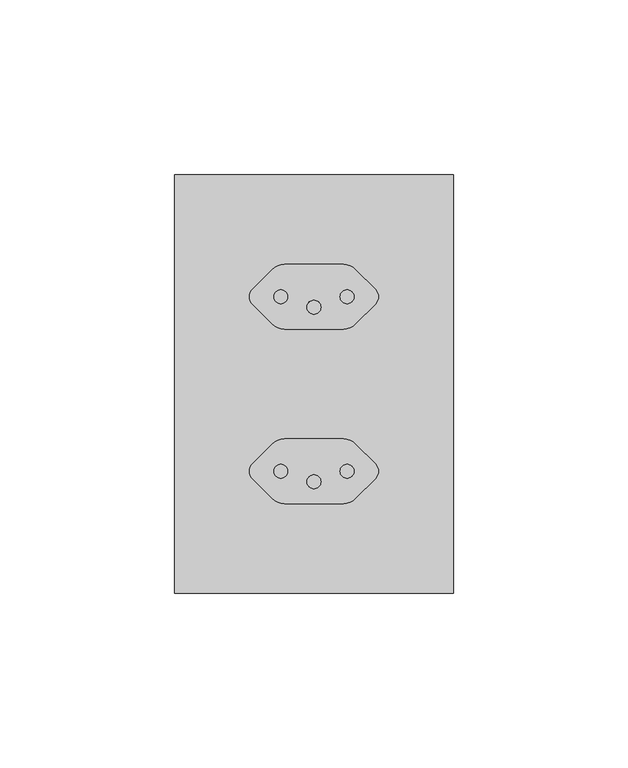
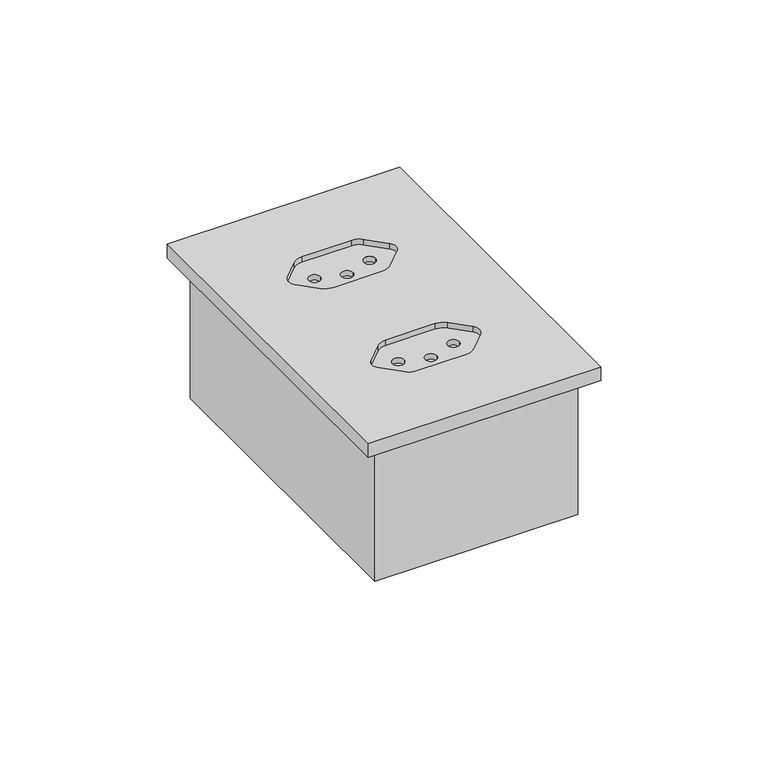
"""IFC4 building model written with IfcOpenShell, lengths in millimetres: proxy geometry, CAIXA VERTICE V7 : Tomada 10A 2s."""

from ifc_helpers import new_model, si_unit, frame, origin, place, context, project, spatial, polyline, circle_curve, faceted_brep, source, transform, mapped, element, save
from ifc_brep_helpers import plane_surface, revolved_surface, advanced_brep


def electrical_fixtures_4c855f6e(model_context):
    return source(origin(), model_context, "Body", "SolidModel", [
        faceted_brep([(33.0, -947.0, -48.0), (-33.0, -947.0, -48.0), (-33.0, -1053.0, -48.0), (33.0, -1053.0, -48.0), (35.0, -1055.0, -50.0), (-35.0, -1055.0, -50.0), (-35.0, -945.0, -50.0), (35.0, -945.0, -50.0), (35.0, -1055.0, 0.0), (-35.0, -1055.0, 0.0), (-35.0, -945.0, 0.0), (35.0, -945.0, 0.0), (33.0, -1053.0, 0.0), (-33.0, -1053.0, 0.0), (-33.0, -947.0, 0.0), (33.0, -947.0, 0.0)], [[[0, 1, 2, 3]], [[4, 5, 6, 7]], [[4, 8, 9, 5]], [[9, 10, 6, 5]], [[10, 11, 7, 6]], [[11, 8, 4, 7]], [[8, 11, 10, 9], [12, 13, 14, 15]], [[15, 0, 3, 12]], [[14, 1, 0, 15]], [[13, 2, 1, 14]], [[12, 3, 2, 13]]]),
        advanced_brep(
        [(40.0, -1060.0, 5.0), (40.0, -940.0, 5.0), (-40.0, -940.0, 5.0), (-40.0, -1060.0, 5.0), (8.4215729, -1015.75, 5.0), (11.9571068, -1017.2144661, 5.0), (17.6213203, -1022.8786797, 5.0), (17.6213203, -1027.1213203, 5.0), (11.9571068, -1032.7855339, 5.0), (8.4215729, -1034.25, 5.0), (-8.4215729, -1034.25, 5.0), (-11.9571068, -1032.7855339, 5.0), (-17.6213203, -1027.1213203, 5.0), (-17.6213203, -1022.8786797, 5.0), (-11.9571068, -1017.2144661, 5.0), (-8.4215729, -1015.75, 5.0), (8.4215729, -965.75, 5.0), (11.9571068, -967.2144661, 5.0), (17.6213203, -972.8786797, 5.0), (17.6213203, -977.1213203, 5.0), (11.9571068, -982.7855339, 5.0), (8.4215729, -984.25, 5.0), (-8.4215729, -984.25, 5.0), (-11.9571068, -982.7855339, 5.0), (-17.6213203, -977.1213203, 5.0), (-17.6213203, -972.8786797, 5.0), (-11.9571068, -967.2144661, 5.0), (-8.4215729, -965.75, 5.0), (-40.0, -1060.0, 0.0), (-40.0, -940.0, 0.0), (40.0, -940.0, 0.0), (40.0, -1060.0, 0.0), (8.4215729, -1015.75, 3.0), (-8.4215729, -1015.75, 3.0), (-11.9571068, -1017.2144661, 3.0), (-17.6213203, -1022.8786797, 3.0), (-17.6213203, -1027.1213203, 3.0), (-11.9571068, -1032.7855339, 3.0), (-8.4215729, -1034.25, 3.0), (8.4215729, -1034.25, 3.0), (11.9571068, -1032.7855339, 3.0), (17.6213203, -1027.1213203, 3.0), (17.6213203, -1022.8786797, 3.0), (11.9571068, -1017.2144661, 3.0), (-7.5, -1025.0, 3.0), (-11.5, -1025.0, 3.0), (11.5, -1025.0, 3.0), (7.5, -1025.0, 3.0), (2.0, -1028.0, 3.0), (-2.0, -1028.0, 3.0), (-11.5, -1025.0, 1.0), (-7.5, -1025.0, 1.0), (7.5, -1025.0, 1.0), (11.5, -1025.0, 1.0), (-2.0, -1028.0, 1.0), (2.0, -1028.0, 1.0), (8.4215729, -965.75, 3.0), (-8.4215729, -965.75, 3.0), (-11.9571068, -967.2144661, 3.0), (-17.6213203, -972.8786797, 3.0), (-17.6213203, -977.1213203, 3.0), (-11.9571068, -982.7855339, 3.0), (-8.4215729, -984.25, 3.0), (8.4215729, -984.25, 3.0), (11.9571068, -982.7855339, 3.0), (17.6213203, -977.1213203, 3.0), (17.6213203, -972.8786797, 3.0), (11.9571068, -967.2144661, 3.0), (-7.5, -975.0, 3.0), (-11.5, -975.0, 3.0), (11.5, -975.0, 3.0), (7.5, -975.0, 3.0), (2.0, -978.0, 3.0), (-2.0, -978.0, 3.0), (-11.5, -975.0, 1.0), (-7.5, -975.0, 1.0), (7.5, -975.0, 1.0), (11.5, -975.0, 1.0), (-2.0, -978.0, 1.0), (2.0, -978.0, 1.0)],
        [
            (0, 1),
            (1, 2),
            (2, 3),
            (3, 0),
            (4, 5, circle_curve(frame((8.4215729, -1020.75, 5.0), z_axis=(0.0, 0.0, -1.0), x_axis=(-1.0, 0.0, 0.0)), 5.0)),
            (5, 6),
            (6, 7, circle_curve(frame((15.5, -1025.0, 5.0), z_axis=(0.0, 0.0, -1.0), x_axis=(-1.0, 0.0, 0.0)), 3.0)),
            (7, 8),
            (8, 9, circle_curve(frame((8.4215729, -1029.25, 5.0), z_axis=(0.0, 0.0, -1.0), x_axis=(-1.0, 0.0, 0.0)), 5.0)),
            (9, 10),
            (10, 11, circle_curve(frame((-8.4215729, -1029.25, 5.0), z_axis=(0.0, 0.0, -1.0), x_axis=(-1.0, 0.0, 0.0)), 5.0)),
            (11, 12),
            (12, 13, circle_curve(frame((-15.5, -1025.0, 5.0), z_axis=(0.0, 0.0, -1.0), x_axis=(-1.0, 0.0, 0.0)), 3.0)),
            (13, 14),
            (14, 15, circle_curve(frame((-8.4215729, -1020.75, 5.0), z_axis=(0.0, 0.0, -1.0), x_axis=(-1.0, 0.0, 0.0)), 5.0)),
            (15, 4),
            (16, 17, circle_curve(frame((8.4215729, -970.75, 5.0), z_axis=(0.0, 0.0, -1.0), x_axis=(-1.0, 0.0, 0.0)), 5.0)),
            (17, 18),
            (18, 19, circle_curve(frame((15.5, -975.0, 5.0), z_axis=(0.0, 0.0, -1.0), x_axis=(-1.0, 0.0, 0.0)), 3.0)),
            (19, 20),
            (20, 21, circle_curve(frame((8.4215729, -979.25, 5.0), z_axis=(0.0, 0.0, -1.0), x_axis=(-1.0, 0.0, 0.0)), 5.0)),
            (21, 22),
            (22, 23, circle_curve(frame((-8.4215729, -979.25, 5.0), z_axis=(0.0, 0.0, -1.0), x_axis=(-1.0, 0.0, 0.0)), 5.0)),
            (23, 24),
            (24, 25, circle_curve(frame((-15.5, -975.0, 5.0), z_axis=(0.0, 0.0, -1.0), x_axis=(-1.0, 0.0, 0.0)), 3.0)),
            (25, 26),
            (26, 27, circle_curve(frame((-8.4215729, -970.75, 5.0), z_axis=(0.0, 0.0, -1.0), x_axis=(-1.0, 0.0, 0.0)), 5.0)),
            (27, 16),
            (28, 29),
            (29, 30),
            (30, 31),
            (31, 28),
            (3, 28),
            (31, 0),
            (2, 29),
            (1, 30),
            (32, 33),
            (33, 34, circle_curve(frame((-8.4215729, -1020.75, 3.0), z_axis=(0.0, 0.0, 1.0), x_axis=(-1.0, 0.0, 0.0)), 5.0)),
            (34, 35),
            (35, 36, circle_curve(frame((-15.5, -1025.0, 3.0), z_axis=(0.0, 0.0, 1.0), x_axis=(-1.0, 0.0, 0.0)), 3.0)),
            (36, 37),
            (37, 38, circle_curve(frame((-8.4215729, -1029.25, 3.0), z_axis=(0.0, 0.0, 1.0), x_axis=(-1.0, 0.0, 0.0)), 5.0)),
            (38, 39),
            (39, 40, circle_curve(frame((8.4215729, -1029.25, 3.0), z_axis=(0.0, 0.0, 1.0), x_axis=(-1.0, 0.0, 0.0)), 5.0)),
            (40, 41),
            (41, 42, circle_curve(frame((15.5, -1025.0, 3.0), z_axis=(0.0, 0.0, 1.0), x_axis=(-1.0, 0.0, 0.0)), 3.0)),
            (42, 43),
            (43, 32, circle_curve(frame((8.4215729, -1020.75, 3.0), z_axis=(0.0, 0.0, 1.0), x_axis=(-1.0, 0.0, 0.0)), 5.0)),
            (44, 45, circle_curve(frame((-9.5, -1025.0, 3.0), z_axis=(0.0, 0.0, -1.0), x_axis=(1.0, -2.301812013077709e-12, 0.0)), 2.0)),
            (45, 44, circle_curve(frame((-9.5, -1025.0, 3.0), z_axis=(0.0, 0.0, -1.0), x_axis=(1.0, -2.301812013077709e-12, 0.0)), 2.0)),
            (46, 47, circle_curve(frame((9.5, -1025.0, 3.0), z_axis=(0.0, 0.0, -1.0), x_axis=(1.0, -2.301812013077709e-12, 0.0)), 2.0)),
            (47, 46, circle_curve(frame((9.5, -1025.0, 3.0), z_axis=(0.0, 0.0, -1.0), x_axis=(1.0, -2.301812013077709e-12, 0.0)), 2.0)),
            (48, 49, circle_curve(frame((0.0, -1028.0, 3.0), z_axis=(0.0, 0.0, -1.0), x_axis=(1.0, -2.301812013077709e-12, 0.0)), 2.0)),
            (49, 48, circle_curve(frame((0.0, -1028.0, 3.0), z_axis=(0.0, 0.0, -1.0), x_axis=(1.0, -2.301812013077709e-12, 0.0)), 2.0)),
            (32, 4),
            (15, 33),
            (14, 34),
            (13, 35),
            (12, 36),
            (11, 37),
            (10, 38),
            (9, 39),
            (8, 40),
            (7, 41),
            (6, 42),
            (5, 43),
            (50, 51, circle_curve(frame((-9.5, -1025.0, 1.0), z_axis=(0.0, 0.0, 1.0), x_axis=(1.0, -2.301812013077709e-12, 0.0)), 2.0)),
            (51, 50, circle_curve(frame((-9.5, -1025.0, 1.0), z_axis=(0.0, 0.0, 1.0), x_axis=(1.0, -2.301812013077709e-12, 0.0)), 2.0)),
            (52, 53, circle_curve(frame((9.5, -1025.0, 1.0), z_axis=(0.0, 0.0, 1.0), x_axis=(1.0, -2.301812013077709e-12, 0.0)), 2.0)),
            (53, 52, circle_curve(frame((9.5, -1025.0, 1.0), z_axis=(0.0, 0.0, 1.0), x_axis=(1.0, -2.301812013077709e-12, 0.0)), 2.0)),
            (54, 55, circle_curve(frame((0.0, -1028.0, 1.0), z_axis=(0.0, 0.0, 1.0), x_axis=(1.0, -2.301812013077709e-12, 0.0)), 2.0)),
            (55, 54, circle_curve(frame((0.0, -1028.0, 1.0), z_axis=(0.0, 0.0, 1.0), x_axis=(1.0, -2.301812013077709e-12, 0.0)), 2.0)),
            (45, 50),
            (51, 44),
            (47, 52),
            (53, 46),
            (49, 54),
            (55, 48),
            (56, 57),
            (57, 58, circle_curve(frame((-8.4215729, -970.75, 3.0), z_axis=(0.0, 0.0, 1.0), x_axis=(-1.0, 0.0, 0.0)), 5.0)),
            (58, 59),
            (59, 60, circle_curve(frame((-15.5, -975.0, 3.0), z_axis=(0.0, 0.0, 1.0), x_axis=(-1.0, 0.0, 0.0)), 3.0)),
            (60, 61),
            (61, 62, circle_curve(frame((-8.4215729, -979.25, 3.0), z_axis=(0.0, 0.0, 1.0), x_axis=(-1.0, 0.0, 0.0)), 5.0)),
            (62, 63),
            (63, 64, circle_curve(frame((8.4215729, -979.25, 3.0), z_axis=(0.0, 0.0, 1.0), x_axis=(-1.0, 0.0, 0.0)), 5.0)),
            (64, 65),
            (65, 66, circle_curve(frame((15.5, -975.0, 3.0), z_axis=(0.0, 0.0, 1.0), x_axis=(-1.0, 0.0, 0.0)), 3.0)),
            (66, 67),
            (67, 56, circle_curve(frame((8.4215729, -970.75, 3.0), z_axis=(0.0, 0.0, 1.0), x_axis=(-1.0, 0.0, 0.0)), 5.0)),
            (68, 69, circle_curve(frame((-9.5, -975.0, 3.0), z_axis=(0.0, 0.0, -1.0), x_axis=(1.0, -2.301812013077709e-12, 0.0)), 2.0)),
            (69, 68, circle_curve(frame((-9.5, -975.0, 3.0), z_axis=(0.0, 0.0, -1.0), x_axis=(1.0, -2.301812013077709e-12, 0.0)), 2.0)),
            (70, 71, circle_curve(frame((9.5, -975.0, 3.0), z_axis=(0.0, 0.0, -1.0), x_axis=(1.0, -2.301812013077709e-12, 0.0)), 2.0)),
            (71, 70, circle_curve(frame((9.5, -975.0, 3.0), z_axis=(0.0, 0.0, -1.0), x_axis=(1.0, -2.301812013077709e-12, 0.0)), 2.0)),
            (72, 73, circle_curve(frame((0.0, -978.0, 3.0), z_axis=(0.0, 0.0, -1.0), x_axis=(1.0, -2.301812013077709e-12, 0.0)), 2.0)),
            (73, 72, circle_curve(frame((0.0, -978.0, 3.0), z_axis=(0.0, 0.0, -1.0), x_axis=(1.0, -2.301812013077709e-12, 0.0)), 2.0)),
            (56, 16),
            (27, 57),
            (26, 58),
            (25, 59),
            (24, 60),
            (23, 61),
            (22, 62),
            (21, 63),
            (20, 64),
            (19, 65),
            (18, 66),
            (17, 67),
            (74, 75, circle_curve(frame((-9.5, -975.0, 1.0), z_axis=(0.0, 0.0, 1.0), x_axis=(1.0, -2.301812013077709e-12, 0.0)), 2.0)),
            (75, 74, circle_curve(frame((-9.5, -975.0, 1.0), z_axis=(0.0, 0.0, 1.0), x_axis=(1.0, -2.301812013077709e-12, 0.0)), 2.0)),
            (76, 77, circle_curve(frame((9.5, -975.0, 1.0), z_axis=(0.0, 0.0, 1.0), x_axis=(1.0, -2.301812013077709e-12, 0.0)), 2.0)),
            (77, 76, circle_curve(frame((9.5, -975.0, 1.0), z_axis=(0.0, 0.0, 1.0), x_axis=(1.0, -2.301812013077709e-12, 0.0)), 2.0)),
            (78, 79, circle_curve(frame((0.0, -978.0, 1.0), z_axis=(0.0, 0.0, 1.0), x_axis=(1.0, -2.301812013077709e-12, 0.0)), 2.0)),
            (79, 78, circle_curve(frame((0.0, -978.0, 1.0), z_axis=(0.0, 0.0, 1.0), x_axis=(1.0, -2.301812013077709e-12, 0.0)), 2.0)),
            (69, 74),
            (75, 68),
            (71, 76),
            (77, 70),
            (73, 78),
            (79, 72),
        ],
        [
            plane_surface(frame((-60.0, -1060.0, 5.0), z_axis=(0.0, 0.0, 1.0), x_axis=(-1.0, 0.0, 0.0))),
            plane_surface(frame((-60.0, -1060.0, 0.0), z_axis=(0.0, 0.0, -1.0), x_axis=(1.0, 0.0, 0.0))),
            plane_surface(frame((40.0, -1060.0, 5.0), z_axis=(0.0, -1.0, 0.0), x_axis=(0.0, 0.0, -1.0))),
            plane_surface(frame((-40.0, -1060.0, 5.0), z_axis=(-1.0, 0.0, 0.0), x_axis=(0.0, 0.0, -1.0))),
            plane_surface(frame((-40.0, -940.0, 5.0), z_axis=(0.0, 1.0, 0.0), x_axis=(0.0, 0.0, -1.0))),
            plane_surface(frame((40.0, -940.0, 5.0), z_axis=(1.0, 0.0, 0.0), x_axis=(0.0, 0.0, -1.0))),
            plane_surface(frame((3.4215729, -1020.75, 3.0), z_axis=(0.0, 0.0, 1.0), x_axis=(0.0, -1.0, 0.0))),
            plane_surface(frame((-8.4215729, -1015.75, 5.0), z_axis=(0.0, -1.0, 0.0), x_axis=(0.0, 0.0, -1.0))),
            revolved_surface(polyline([(-13.4215729, -1020.75, 5.0), (-13.4215729, -1020.75, 3.0)]), (-8.4215729, -1020.75, 3.0), (0.0, 0.0, 1.0)),
            plane_surface(frame((-17.6213203, -1022.8786797, 5.0), z_axis=(0.7071067811865045, -0.7071067811865905, 0.0), x_axis=(0.0, 0.0, -1.0))),
            revolved_surface(polyline([(-18.5, -1025.0, 5.0), (-18.5, -1025.0, 3.0)]), (-15.5, -1025.0, 3.0), (0.0, 0.0, 1.0)),
            plane_surface(frame((-11.9571068, -1032.7855339, 5.0), z_axis=(0.7071067811865515, 0.7071067811865437, 0.0), x_axis=(0.0, 0.0, -1.0))),
            revolved_surface(polyline([(-13.4215729, -1029.25, 5.0), (-13.4215729, -1029.25, 3.0)]), (-8.4215729, -1029.25, 3.0), (0.0, 0.0, 1.0)),
            plane_surface(frame((8.4215729, -1034.25, 5.0), z_axis=(0.0, 1.0, 0.0), x_axis=(0.0, 0.0, -1.0))),
            revolved_surface(polyline([(3.4215728999999993, -1029.25, 5.0), (3.4215728999999993, -1029.25, 3.0)]), (8.4215729, -1029.25, 3.0), (0.0, 0.0, 1.0)),
            plane_surface(frame((17.6213203, -1027.1213203, 5.0), z_axis=(-0.7071067811865307, 0.7071067811865643, 0.0), x_axis=(0.0, 0.0, -1.0))),
            revolved_surface(polyline([(12.5, -1025.0, 5.0), (12.5, -1025.0, 3.0)]), (15.5, -1025.0, 3.0), (0.0, 0.0, 1.0)),
            plane_surface(frame((11.9571068, -1017.2144661, 5.0), z_axis=(-0.7071067811865893, -0.7071067811865058, 0.0), x_axis=(0.0, 0.0, -1.0))),
            revolved_surface(polyline([(3.4215728999999993, -1020.75, 5.0), (3.4215728999999993, -1020.75, 3.0)]), (8.4215729, -1020.75, 3.0), (0.0, 0.0, 1.0)),
            plane_surface(frame((-7.5, -1025.0, 1.0), z_axis=(0.0, 0.0, 1.0), x_axis=(2.301812013077709e-12, 1.0, 0.0))),
            revolved_surface(polyline([(-7.5, -1025.0000000000045, 3.0), (-7.5, -1025.0000000000045, 1.0)]), (-9.5, -1025.0, 1.0), (0.0, 0.0, 1.0)),
            revolved_surface(polyline([(11.5, -1025.0000000000045, 3.0), (11.5, -1025.0000000000045, 1.0)]), (9.5, -1025.0, 5.0), (0.0, 0.0, 1.0)),
            revolved_surface(polyline([(2.0, -1028.0000000000045, 3.0), (2.0, -1028.0000000000045, 1.0)]), (0.0, -1028.0, 5.0), (0.0, 0.0, 1.0)),
            plane_surface(frame((3.4215729, -970.75, 3.0), z_axis=(0.0, 0.0, 1.0), x_axis=(0.0, -1.0, 0.0))),
            plane_surface(frame((-8.4215729, -965.75, 5.0), z_axis=(0.0, -1.0, 0.0), x_axis=(0.0, 0.0, -1.0))),
            revolved_surface(polyline([(-13.4215729, -970.75, 5.0), (-13.4215729, -970.75, 3.0)]), (-8.4215729, -970.75, 3.0), (0.0, 0.0, 1.0)),
            plane_surface(frame((-17.6213203, -972.8786797, 5.0), z_axis=(0.7071067811865045, -0.7071067811865905, 0.0), x_axis=(0.0, 0.0, -1.0))),
            revolved_surface(polyline([(-18.5, -975.0, 5.0), (-18.5, -975.0, 3.0)]), (-15.5, -975.0, 3.0), (0.0, 0.0, 1.0)),
            plane_surface(frame((-11.9571068, -982.7855339, 5.0), z_axis=(0.7071067811865515, 0.7071067811865437, 0.0), x_axis=(0.0, 0.0, -1.0))),
            revolved_surface(polyline([(-13.4215729, -979.25, 5.0), (-13.4215729, -979.25, 3.0)]), (-8.4215729, -979.25, 3.0), (0.0, 0.0, 1.0)),
            plane_surface(frame((8.4215729, -984.25, 5.0), z_axis=(0.0, 1.0, 0.0), x_axis=(0.0, 0.0, -1.0))),
            revolved_surface(polyline([(3.4215728999999993, -979.25, 5.0), (3.4215728999999993, -979.25, 3.0)]), (8.4215729, -979.25, 3.0), (0.0, 0.0, 1.0)),
            plane_surface(frame((17.6213203, -977.1213203, 5.0), z_axis=(-0.7071067811865307, 0.7071067811865643, 0.0), x_axis=(0.0, 0.0, -1.0))),
            revolved_surface(polyline([(12.5, -975.0, 5.0), (12.5, -975.0, 3.0)]), (15.5, -975.0, 3.0), (0.0, 0.0, 1.0)),
            plane_surface(frame((11.9571068, -967.2144661, 5.0), z_axis=(-0.7071067811865893, -0.7071067811865058, 0.0), x_axis=(0.0, 0.0, -1.0))),
            revolved_surface(polyline([(3.4215728999999993, -970.75, 5.0), (3.4215728999999993, -970.75, 3.0)]), (8.4215729, -970.75, 3.0), (0.0, 0.0, 1.0)),
            plane_surface(frame((-7.5, -975.0, 1.0), z_axis=(0.0, 0.0, 1.0), x_axis=(2.301812013077709e-12, 1.0, 0.0))),
            revolved_surface(polyline([(-7.5, -975.0000000000045, 3.0), (-7.5, -975.0000000000045, 1.0)]), (-9.5, -975.0, 1.0), (0.0, 0.0, 1.0)),
            revolved_surface(polyline([(11.5, -975.0000000000045, 3.0), (11.5, -975.0000000000045, 1.0)]), (9.5, -975.0, 5.0), (0.0, 0.0, 1.0)),
            revolved_surface(polyline([(2.0, -978.0000000000045, 3.0), (2.0, -978.0000000000045, 1.0)]), (0.0, -978.0, 5.0), (0.0, 0.0, 1.0)),
        ],
        [
            (0, [[1, 2, 3, 4], [5, 6, 7, 8, 9, 10, 11, 12, 13, 14, 15, 16], [17, 18, 19, 20, 21, 22, 23, 24, 25, 26, 27, 28]]),
            (1, [[29, 30, 31, 32]]),
            (2, [[33, -32, 34, -4]]),
            (3, [[35, -29, -33, -3]]),
            (4, [[36, -30, -35, -2]]),
            (5, [[-34, -31, -36, -1]]),
            (6, [[37, 38, 39, 40, 41, 42, 43, 44, 45, 46, 47, 48], [49, 50], [51, 52], [53, 54]]),
            (7, [[55, -16, 56, -37]]),
            (8, [[-56, -15, 57, -38]]),
            (9, [[-57, -14, 58, -39]]),
            (10, [[-58, -13, 59, -40]]),
            (11, [[-59, -12, 60, -41]]),
            (12, [[-60, -11, 61, -42]]),
            (13, [[-61, -10, 62, -43]]),
            (14, [[-62, -9, 63, -44]]),
            (15, [[-63, -8, 64, -45]]),
            (16, [[-64, -7, 65, -46]]),
            (17, [[-65, -6, 66, -47]]),
            (18, [[-66, -5, -55, -48]]),
            (19, [[67, 68]]),
            (19, [[69, 70]]),
            (19, [[71, 72]]),
            (20, [[73, -68, 74, -50]]),
            (20, [[-74, -67, -73, -49]]),
            (21, [[75, -70, 76, -52]]),
            (21, [[-76, -69, -75, -51]]),
            (22, [[77, -72, 78, -54]]),
            (22, [[-78, -71, -77, -53]]),
            (23, [[79, 80, 81, 82, 83, 84, 85, 86, 87, 88, 89, 90], [91, 92], [93, 94], [95, 96]]),
            (24, [[97, -28, 98, -79]]),
            (25, [[-98, -27, 99, -80]]),
            (26, [[-99, -26, 100, -81]]),
            (27, [[-100, -25, 101, -82]]),
            (28, [[-101, -24, 102, -83]]),
            (29, [[-102, -23, 103, -84]]),
            (30, [[-103, -22, 104, -85]]),
            (31, [[-104, -21, 105, -86]]),
            (32, [[-105, -20, 106, -87]]),
            (33, [[-106, -19, 107, -88]]),
            (34, [[-107, -18, 108, -89]]),
            (35, [[-108, -17, -97, -90]]),
            (36, [[109, 110]]),
            (36, [[111, 112]]),
            (36, [[113, 114]]),
            (37, [[115, -110, 116, -92]]),
            (37, [[-116, -109, -115, -91]]),
            (38, [[117, -112, 118, -94]]),
            (38, [[-118, -111, -117, -93]]),
            (39, [[119, -114, 120, -96]]),
            (39, [[-120, -113, -119, -95]]),
        ],
    ),
    ])


if __name__ == "__main__":
    model = new_model("IFC4")
    model_context = context("Model", 3, world=origin())
    ifc_project = project(units=[si_unit("LENGTHUNIT", "METRE", prefix="MILLI")], contexts=[model_context])
    site = spatial("IfcSite", under=ifc_project)
    building = spatial("IfcBuilding", under=site)
    placement = place(None, origin())
    electrical_fixtures_shape = electrical_fixtures_4c855f6e(model_context)
    element("IfcBuildingElementProxy", 1, Name="CAIXA VERTICE V7 : Tomada 10A 2s", ObjectType="CAIXA VERTICE V7 : Tomada 10A 2s", at=placement, inside=building, context=model_context, shape_type="MappedRepresentation", body=[
        mapped(electrical_fixtures_shape, transform((0.0, 0.0, 0.0), x_axis=(1.0, 0.0, 0.0), y_axis=(0.0, 1.0, 0.0), z_axis=(0.0, 0.0, 1.0))),
    ])
    save(model, "model.ifc")

# Revit data of these elements
# Type "CAIXA VERTICE V7 : Tomada 10A 2s"
#   URL = "www.facebook.com/verticetreinamentos"
#   SEÇÃO [instance default] = ""
#   Rotação [instance default] = 0.00°
#   LARGURA DA TAMPA = 0.08 m
#   BORDA = 0.01 m
#   ALTURA DE INSTALAÇÃO [instance default] = 1.10 m
#   Distância Anotação [instance default] = 0.0015 m
#   ALTURA DA TAMPA = 0.12 m
#   Vertical [instance default] = yes
#   VER SEÇÃO [instance default] = no
#   SHADE ESQ [instance default] = no
#   SHADE DIR [instance default] = yes
#   HORIZONTAL [instance default] = no
#   ANDAR COM A LEGENDA [instance default] = 0
#   Material Tampa [instance default] = Plástico, branco opaco
#   Caixa = element 1798515
#   Anotação = element 1798529
#   Default Elevation = 0
# Element 1 (IfcBuildingElementProxy, "CAIXA VERTICE V7 : Tomada 10A 2s")
#   ALTURA DE INSTALAÇÃO = 1.00 m
#   Materials on its faces: "Plástico, branco opaco"
# Materials
#   "Plástico, branco opaco": class "Plástico", colour RGB 120 120 120, transparency 0, Description = "Plastic, generic, opaque white", Cost = 0
